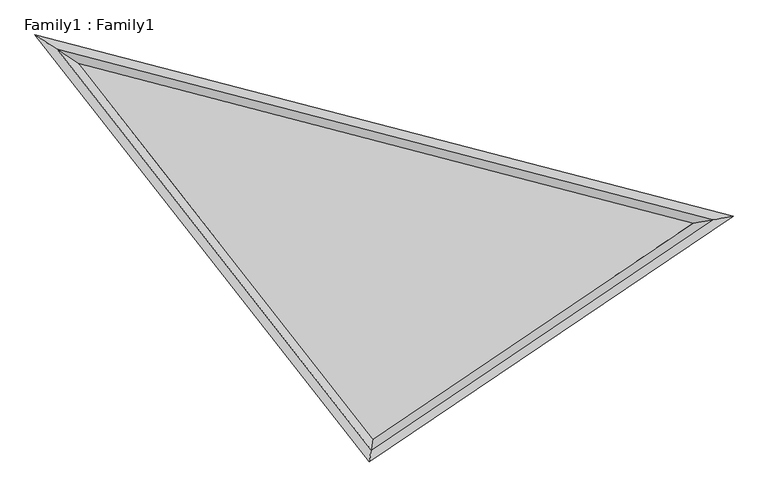
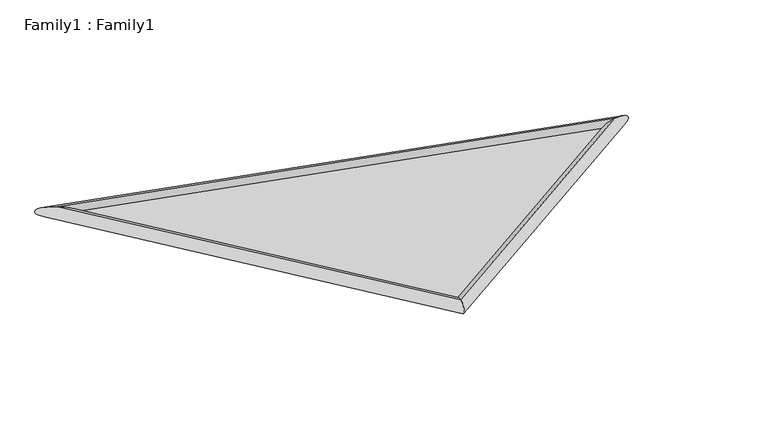
"""IFC4 building model written with IfcOpenShell, lengths in millimetres: proxy geometry, Family1 : Family1."""

from ifc_helpers import new_model, si_unit, frame, origin, origin_with_axes, place, context, project, spatial, polyline, ellipse_curve, outline, extrude, source, transform, mapped, element, save
from ifc_brep_helpers import cylinder_surface, advanced_brep


def family1_family1_db3dfae6(model_context):
    return source(origin(), model_context, "Body", "SolidModel", [
        extrude(outline(polyline([(815.617667, -1995.0287102), (-2850.8862136, 2684.0678402), (4802.1909975, 694.9020749), (815.617667, -1995.0287102)])), origin_with_axes(), (0.0, 0.0, 1.0), 34.1328789),
        advanced_brep(
        [(815.617667, -1995.0287102, 100.0), (815.617667, -1995.0287102, -100.0), (-2850.8862136, 2684.0678402, -100.0), (-2850.8862136, 2684.0678402, 100.0), (4802.1909975, 694.9020749, -100.0), (4802.1909975, 694.9020749, 100.0)],
        [
            (0, 1, ellipse_curve(frame((815.617667, -1995.0287102, 0.0), z_axis=(-0.9878127858326851, 0.15564671581973638, 0.0), x_axis=(-0.15564671581973644, -0.9878127858326851, 0.0)), 136.6520829, 100.0)),
            (1, 2),
            (2, 3, ellipse_curve(frame((-2850.8862136, 2684.0678402, 0.0), z_axis=(-0.5482041402196806, -0.8363445585678195, 0.0), x_axis=(0.8363445585678195, -0.5482041402196804, 0.0)), 312.3191938, 100.0)),
            (3, 0),
            (1, 0, ellipse_curve(frame((815.617667, -1995.0287102, 0.0), z_axis=(-0.9878127858326851, 0.15564671581973638, 0.0), x_axis=(-0.15564671581973644, -0.9878127858326851, 0.0)), 136.6520829, 100.0)),
            (3, 2, ellipse_curve(frame((-2850.8862136, 2684.0678402, 0.0), z_axis=(-0.5482041402196806, -0.8363445585678195, 0.0), x_axis=(0.8363445585678195, -0.5482041402196804, 0.0)), 312.3191938, 100.0)),
            (2, 4),
            (4, 5, ellipse_curve(frame((4802.1909975, 694.9020749, 0.0), z_axis=(-0.16883039957850535, 0.9856451167525573, 0.0), x_axis=(-0.9856451167525573, -0.1688303995785054, 0.0)), 243.1027052, 100.0)),
            (5, 3),
            (5, 4, ellipse_curve(frame((4802.1909975, 694.9020749, 0.0), z_axis=(-0.16883039957850535, 0.9856451167525573, 0.0), x_axis=(-0.9856451167525573, -0.1688303995785054, 0.0)), 243.1027052, 100.0)),
            (4, 1),
            (0, 5),
        ],
        [
            cylinder_surface(frame((815.617667, -1995.0287102, 0.0), z_axis=(0.6167882774506652, -0.7871291004653819, 0.0), x_axis=(-0.7871291004653819, -0.6167882774506652, 0.0)), 100.0),
            cylinder_surface(frame((-2850.8862136, 2684.0678402, 0.0), z_axis=(-0.9678420398153204, 0.25155871276129543, 0.0), x_axis=(0.25155871276129543, 0.9678420398153204, 0.0)), 100.0),
            cylinder_surface(frame((4802.1909975, 694.9020749, 0.0), z_axis=(0.8289456836758322, 0.5593291101982868, 0.0), x_axis=(0.5593291101982868, -0.8289456836758322, 0.0)), 100.0),
        ],
        [
            (0, [[1, 2, 3, 4]]),
            (0, [[5, -4, 6, -2]]),
            (1, [[-3, 7, 8, 9]]),
            (1, [[-6, -9, 10, -7]]),
            (2, [[-8, 11, -1, 12]]),
            (2, [[-10, -12, -5, -11]]),
        ],
    ),
    ])


if __name__ == "__main__":
    model = new_model("IFC4")
    model_context = context("Model", 3, world=origin())
    ifc_project = project(units=[si_unit("LENGTHUNIT", "METRE", prefix="MILLI")], contexts=[model_context])
    site = spatial("IfcSite", under=ifc_project)
    building = spatial("IfcBuilding", under=site)
    placement = place(None, origin())
    family1_family1_shape = family1_family1_db3dfae6(model_context)
    element("IfcBuildingElementProxy", 1, Name="Family1 : Family1", ObjectType="Family1 : Family1", at=placement, inside=building, context=model_context, shape_type="MappedRepresentation", body=[
        mapped(family1_family1_shape, transform((0.0, 0.0, 0.0), x_axis=(1.0, 0.0, 0.0), y_axis=(0.0, 1.0, 0.0), z_axis=(0.0, 0.0, 1.0))),
    ])
    save(model, "model.ifc")

# Revit data of these elements
# Type "Family1 : Family1"
#   Default Elevation = 0
# Element 1 (IfcBuildingElementProxy, "Family1 : Family1")
#   Materials on its faces: "Glass"
# Materials
#   "Glass": class "Glass", colour RGB 0 128 192, transparency 0.9, Description = "Soda Lime Glass", Cost = 0
